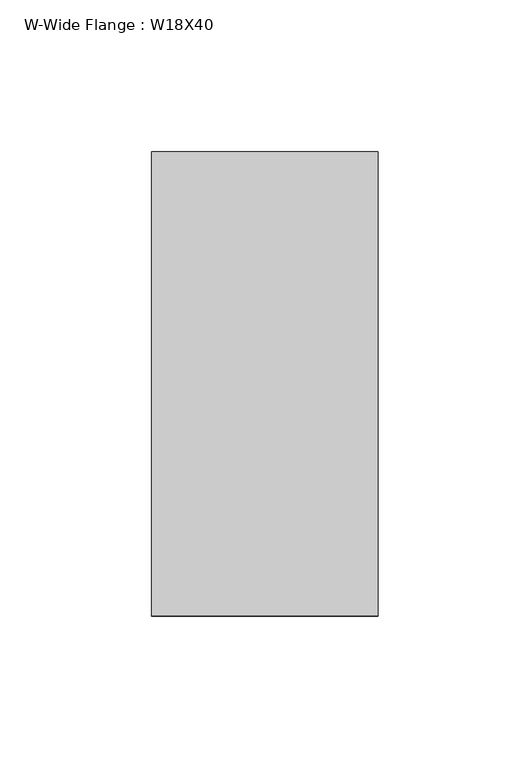
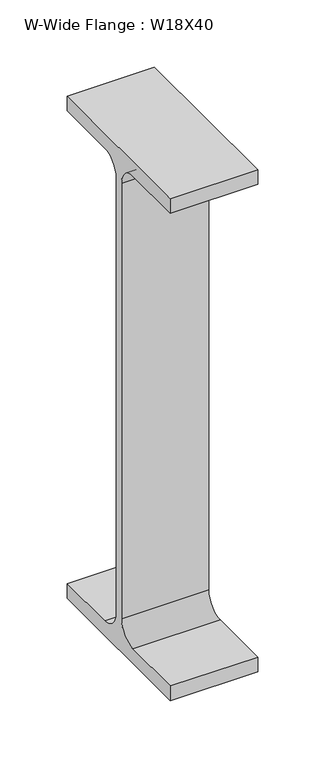
"""IFC4 building model written with IfcOpenShell, lengths in millimetres: beam geometry, W-Wide Flange : W18X40."""

import ifcopenshell
import ifcopenshell.guid

model = None  # the IFC model being written
_history = None  # IfcOwnerHistory: only IFC2X3 demands one
_inside = {}  # id of a spatial element -> (the spatial element, [elements in it])
_under = {}  # id of a project, library or spatial element -> (it, [spatial elements below it])
_declared = {}  # id of a project -> (the project, [libraries it declares])
_typed = {}  # id of a type object -> (the type object, [elements of that type])
_made_of = {}  # id of a material, layer set ... -> (it, [elements and type objects made of it])


def new_model(schema):
    """Start an empty IFC model of exactly this schema.

    Asked for "IFC4X3", IfcOpenShell would pick the latest addendum, in which some entities
    have other attributes; the version numbers below select the first issue.
    IFC2X3 requires an IfcOwnerHistory on every rooted entity: one is made here for all.
    """
    global model, _history
    if schema == "IFC4X3":
        model = ifcopenshell.file(schema_version=(4, 3, 0, 0))
    else:
        model = ifcopenshell.file(schema=schema)
    _inside.clear()
    _under.clear()
    _declared.clear()
    _typed.clear()
    _made_of.clear()
    _history = None
    if model.schema == "IFC2X3":
        org = make("IfcOrganization", Name="unknown")
        user = make(
            "IfcPersonAndOrganization",
            ThePerson=make("IfcPerson", FamilyName="unknown"),
            TheOrganization=org,
        )
        app = make(
            "IfcApplication",
            ApplicationDeveloper=org,
            Version="unknown",
            ApplicationFullName="unknown",
            ApplicationIdentifier="unknown",
        )
        _history = make(
            "IfcOwnerHistory",
            OwningUser=user,
            OwningApplication=app,
            ChangeAction="ADDED",
            CreationDate=0,
        )
    return model


def make(cls, **values):
    """One entity of the class cls with the attributes given. An attribute that is None is left unset."""
    return model.create_entity(
        cls, **{name: value for name, value in values.items() if value is not None}
    )


def rooted(cls, **values):
    """An entity with a GlobalId (a new one), such as an element, a storey or a relation."""
    return make(cls, GlobalId=ifcopenshell.guid.new(), OwnerHistory=_history, **values)


def si_unit(unit_type, name, prefix=None):
    """IfcSIUnit, for example si_unit("LENGTHUNIT", "METRE", prefix="MILLI")."""
    return make("IfcSIUnit", UnitType=unit_type, Prefix=prefix, Name=name)


def assignment(units):
    """IfcUnitAssignment: the units of a project."""
    return None if units is None else make("IfcUnitAssignment", Units=units)


def point(xyz):
    """IfcCartesianPoint."""
    return None if xyz is None else make("IfcCartesianPoint", Coordinates=xyz)


def direction(xyz):
    """IfcDirection."""
    return None if xyz is None else make("IfcDirection", DirectionRatios=xyz)


def frame(location, z_axis=None, x_axis=None):
    """IfcAxis2Placement3D, a coordinate frame: its origin and axes. An axis left out is left unset."""
    return make(
        "IfcAxis2Placement3D",
        Location=point(location),
        Axis=direction(z_axis),
        RefDirection=direction(x_axis),
    )


def frame_2d(location, x_axis=None):
    """IfcAxis2Placement2D, a coordinate frame in the plane: its origin and x axis."""
    return make(
        "IfcAxis2Placement2D", Location=point(location), RefDirection=direction(x_axis)
    )


def origin():
    """The frame at (0, 0, 0) with its axes left unset."""
    return frame((0.0, 0.0, 0.0))


def place(relative_to, where):
    """IfcLocalPlacement: puts the frame where relative to a parent placement (None: the world)."""
    return make(
        "IfcLocalPlacement", PlacementRelTo=relative_to, RelativePlacement=where
    )


def context(
    kind, dimensions, precision=None, world=None, true_north=None, identifier=None
):
    """IfcGeometricRepresentationContext, for example the 3D "Model" context."""
    return make(
        "IfcGeometricRepresentationContext",
        ContextIdentifier=identifier,
        ContextType=kind,
        CoordinateSpaceDimension=dimensions,
        Precision=precision,
        WorldCoordinateSystem=world,
        TrueNorth=true_north,
    )


def project(units=None, contexts=None):
    """IfcProject with its units and contexts."""
    return rooted(
        "IfcProject",
        Name="project",
        RepresentationContexts=contexts,
        UnitsInContext=assignment(units),
    )


def spatial(cls, under=None, at=None, **own):
    """A site, building, storey or space (cls), placed at a placement, below another one or the project."""
    s = rooted(cls, ObjectPlacement=at, **own)
    if under is not None:
        _under.setdefault(under.id(), (under, []))[1].append(s)
    return s


def polyline(points):
    """IfcPolyline through the points."""
    return make("IfcPolyline", Points=[point(p) for p in points])


def circle_curve(where, radius):
    """IfcCircle in the frame where."""
    return make("IfcCircle", Position=where, Radius=radius)


def trimmed(basis, trim1, trim2, sense, master):
    """IfcTrimmedCurve: the piece of a basis curve between two trims."""
    return make(
        "IfcTrimmedCurve",
        BasisCurve=basis,
        Trim1=trim1,
        Trim2=trim2,
        SenseAgreement=sense,
        MasterRepresentation=master,
    )


def segment(curve, same_sense, transition):
    """IfcCompositeCurveSegment."""
    return make(
        "IfcCompositeCurveSegment",
        Transition=transition,
        SameSense=same_sense,
        ParentCurve=curve,
    )


def composite_curve(segments, self_intersect=None):
    """IfcCompositeCurve: segments joined end to end."""
    return make("IfcCompositeCurve", Segments=segments, SelfIntersect=self_intersect)


def outline(outer, holes=None, kind="AREA"):
    """IfcArbitraryClosedProfileDef: a profile drawn as a closed curve; with holes, ...WithVoids."""
    if holes is None:
        return make("IfcArbitraryClosedProfileDef", ProfileType=kind, OuterCurve=outer)
    return make(
        "IfcArbitraryProfileDefWithVoids",
        ProfileType=kind,
        OuterCurve=outer,
        InnerCurves=holes,
    )


def extrude(swept, where, along, depth):
    """IfcExtrudedAreaSolid: the profile swept, set in the frame where, extruded along a direction by depth."""
    return make(
        "IfcExtrudedAreaSolid",
        SweptArea=swept,
        Position=where,
        ExtrudedDirection=direction(along),
        Depth=depth,
    )


def shape(context_of_items, identifier, shape_type, items):
    """IfcShapeRepresentation: the items that make up one representation, for example the "Body"."""
    return make(
        "IfcShapeRepresentation",
        ContextOfItems=context_of_items,
        RepresentationIdentifier=identifier,
        RepresentationType=shape_type,
        Items=items,
    )


def source(mapping_origin, context_of_items, identifier, shape_type, items):
    """IfcRepresentationMap: a shape defined once, which mapped items show again and again."""
    return make(
        "IfcRepresentationMap",
        MappingOrigin=mapping_origin,
        MappedRepresentation=shape(context_of_items, identifier, shape_type, items),
    )


def transform(
    local_origin,
    x_axis=None,
    y_axis=None,
    z_axis=None,
    scale=None,
    scale2=None,
    scale3=None,
    uniform=True,
):
    """IfcCartesianTransformationOperator3D, or its non-uniform kind. x_axis, y_axis, z_axis: its Axis1, 2, 3."""
    if uniform:
        return make(
            "IfcCartesianTransformationOperator3D",
            Axis1=direction(x_axis),
            Axis2=direction(y_axis),
            LocalOrigin=point(local_origin),
            Scale=scale,
            Axis3=direction(z_axis),
        )
    return make(
        "IfcCartesianTransformationOperator3DnonUniform",
        Axis1=direction(x_axis),
        Axis2=direction(y_axis),
        LocalOrigin=point(local_origin),
        Scale=scale,
        Axis3=direction(z_axis),
        Scale2=scale2,
        Scale3=scale3,
    )


def mapped(mapping_source, mapping_target):
    """IfcMappedItem: shows the shape of a source again, moved by a transform."""
    return make(
        "IfcMappedItem", MappingSource=mapping_source, MappingTarget=mapping_target
    )


def made_of(thing, what):
    """Note that an element or type object is made of a material, layer set ...; save() writes the relation."""
    if what is not None:
        _made_of.setdefault(what.id(), (what, []))[1].append(thing)
    return thing


def element(
    cls,
    number,
    at=None,
    inside=None,
    cuts=None,
    type_object=None,
    material=None,
    context=None,
    identifier="Body",
    shape_type=None,
    held_by="IfcProductDefinitionShape",
    body=None,
    shapes=None,
    **own,
):
    """One element of the class cls, such as IfcWall. Its Tag is "e" and its number.

    at: its placement. inside: the storey or other place that contains it. cuts: it is an
    opening in that element (IfcRelVoidsElement). A single representation is given by context,
    identifier, shape_type and body (its items); several are given by shapes. held_by: the class
    of the entity that holds the representations. save() writes the other relations.
    """
    e = rooted(cls, Tag="e%d" % number, ObjectPlacement=at, **own)
    if body is not None:
        shapes = [shape(context, identifier, shape_type, body)]
    if shapes is not None:
        e.Representation = make(held_by, Representations=shapes)
    if inside is not None:
        _inside.setdefault(inside.id(), (inside, []))[1].append(e)
    if cuts is not None:
        rooted(
            "IfcRelVoidsElement", RelatingBuildingElement=cuts, RelatedOpeningElement=e
        )
    if type_object is not None:
        _typed.setdefault(type_object.id(), (type_object, []))[1].append(e)
    return made_of(e, material)


def aggregate(whole, parts):
    """IfcRelAggregates: a whole, such as a stair, and the parts it consists of."""
    return rooted("IfcRelAggregates", RelatingObject=whole, RelatedObjects=parts)


def save(model, path):
    """Write the relations noted so far, then the file.

    IfcRelAggregates (storeys below a building ...), IfcRelContainedInSpatialStructure (elements
    in a storey), IfcRelDefinesByType, IfcRelAssociatesMaterial and IfcRelDeclares: one each for
    every whole, place, type object, material and project.
    """
    for whole, parts in _under.values():
        aggregate(whole, parts)
    for where, things in _inside.values():
        rooted(
            "IfcRelContainedInSpatialStructure",
            RelatedElements=things,
            RelatingStructure=where,
        )
    for kind, things in _typed.values():
        rooted("IfcRelDefinesByType", RelatedObjects=things, RelatingType=kind)
    for what, things in _made_of.values():
        rooted("IfcRelAssociatesMaterial", RelatedObjects=things, RelatingMaterial=what)
    for by, libraries in _declared.values():
        rooted("IfcRelDeclares", RelatingContext=by, RelatedDefinitions=libraries)
    model.write(path)


def w_wide_flange_w18x40_776be871(model_context):
    return source(origin(), model_context, "Body", "SweptSolid", [
        extrude(outline(composite_curve([segment(polyline([(76.454, -213.995), (76.454, -227.33), (-76.454, -227.33), (-76.454, -213.995), (-20.828, -213.995)]), True, "CONTINUOUS"), segment(trimmed(circle_curve(frame_2d((-20.828, -197.1675)), 16.8275), [point((-20.828, -213.995))], [point((-4.0005, -197.1675))], True, "CARTESIAN"), True, "CONTINUOUS"), segment(polyline([(-4.0005, -197.1675), (-4.0005, 197.1675)]), True, "CONTINUOUS"), segment(trimmed(circle_curve(frame_2d((-20.828, 197.1675)), 16.8275), [point((-4.0005, 197.1675))], [point((-20.828, 213.995))], True, "CARTESIAN"), True, "CONTINUOUS"), segment(polyline([(-20.828, 213.995), (-76.454, 213.995), (-76.454, 227.33), (76.454, 227.33), (76.454, 213.995), (20.828, 213.995)]), True, "CONTINUOUS"), segment(trimmed(circle_curve(frame_2d((20.828, 197.1675)), 16.8275), [point((20.828, 213.995))], [point((4.0005, 197.1675))], True, "CARTESIAN"), True, "CONTINUOUS"), segment(polyline([(4.0005, 197.1675), (4.0005, -197.1675)]), True, "CONTINUOUS"), segment(trimmed(circle_curve(frame_2d((20.828, -197.1675)), 16.8275), [point((4.0005, -197.1675))], [point((20.828, -213.995))], True, "CARTESIAN"), True, "CONTINUOUS"), segment(polyline([(20.828, -213.995), (76.454, -213.995)]), True, "CONTINUOUS")], self_intersect=False)), frame((-68.2625, 0.0, 0.0), z_axis=(1.0, 0.0, 0.0), x_axis=(0.0, 1.0, 0.0)), (0.0, 0.0, 1.0), 74.6125),
    ])


if __name__ == "__main__":
    model = new_model("IFC4")
    model_context = context("Model", 3, world=origin())
    ifc_project = project(units=[si_unit("LENGTHUNIT", "METRE", prefix="MILLI")], contexts=[model_context])
    site = spatial("IfcSite", under=ifc_project)
    building = spatial("IfcBuilding", under=site)
    placement = place(None, origin())
    w_wide_flange_w18x40_shape = w_wide_flange_w18x40_776be871(model_context)
    element("IfcBeam", 1, ObjectType="W-Wide Flange : W18X40", at=placement, inside=building, context=model_context, shape_type="MappedRepresentation", body=[
        mapped(w_wide_flange_w18x40_shape, transform((0.0, 0.0, 0.0), x_axis=(1.0, 0.0, 0.0), y_axis=(0.0, 1.0, 0.0), z_axis=(0.0, 0.0, 1.0))),
    ])
    save(model, "model.ifc")

# Revit data of these elements
# Type "W-Wide Flange : W18X40"
#   Assembly Code = "B10"
#   W = 40
#   Length [instance default] = 5' - 0"
#   bf = 0' - 6.02"
#   d = 1' - 5.9"
#   k = 0' - 1 3/16"
#   k2 = 0' - 0.6625"
#   tf = 0' - 0.525"
#   tw = 0' - 0.315"
#   A = 0.0819444 SF
#   Structural Material [instance default] = Steel ASTM A992
# Element 1 (IfcBeam, "W-Wide Flange : W18X40")
#   Materials on its faces: "Steel ASTM A992"
# Materials
#   "Steel ASTM A992": class "Metal", colour RGB 199 199 199, transparency 0, Description = "Structural steel 50ksi", Cost = 0
